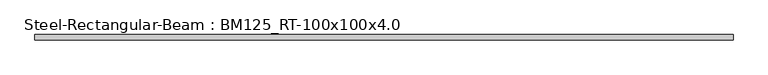
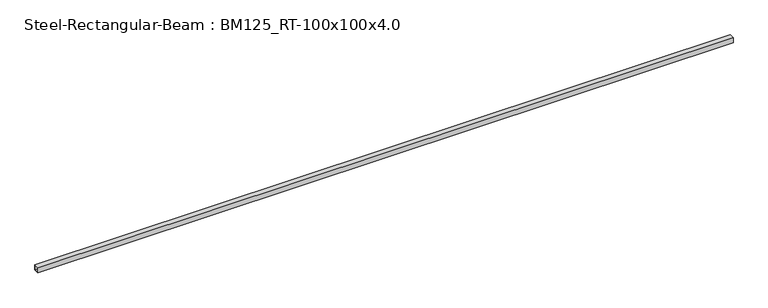
"""IFC4 building model written with IfcOpenShell, lengths in millimetres: beam geometry, Steel-Rectangular-Beam : BM125_RT-100x100x4.0."""

import ifcopenshell
import ifcopenshell.guid

model = None  # the IFC model being written
_history = None  # IfcOwnerHistory: only IFC2X3 demands one
_inside = {}  # id of a spatial element -> (the spatial element, [elements in it])
_under = {}  # id of a project, library or spatial element -> (it, [spatial elements below it])
_declared = {}  # id of a project -> (the project, [libraries it declares])
_typed = {}  # id of a type object -> (the type object, [elements of that type])
_made_of = {}  # id of a material, layer set ... -> (it, [elements and type objects made of it])


def new_model(schema):
    """Start an empty IFC model of exactly this schema.

    Asked for "IFC4X3", IfcOpenShell would pick the latest addendum, in which some entities
    have other attributes; the version numbers below select the first issue.
    IFC2X3 requires an IfcOwnerHistory on every rooted entity: one is made here for all.
    """
    global model, _history
    if schema == "IFC4X3":
        model = ifcopenshell.file(schema_version=(4, 3, 0, 0))
    else:
        model = ifcopenshell.file(schema=schema)
    _inside.clear()
    _under.clear()
    _declared.clear()
    _typed.clear()
    _made_of.clear()
    _history = None
    if model.schema == "IFC2X3":
        org = make("IfcOrganization", Name="unknown")
        user = make(
            "IfcPersonAndOrganization",
            ThePerson=make("IfcPerson", FamilyName="unknown"),
            TheOrganization=org,
        )
        app = make(
            "IfcApplication",
            ApplicationDeveloper=org,
            Version="unknown",
            ApplicationFullName="unknown",
            ApplicationIdentifier="unknown",
        )
        _history = make(
            "IfcOwnerHistory",
            OwningUser=user,
            OwningApplication=app,
            ChangeAction="ADDED",
            CreationDate=0,
        )
    return model


def make(cls, **values):
    """One entity of the class cls with the attributes given. An attribute that is None is left unset."""
    return model.create_entity(
        cls, **{name: value for name, value in values.items() if value is not None}
    )


def rooted(cls, **values):
    """An entity with a GlobalId (a new one), such as an element, a storey or a relation."""
    return make(cls, GlobalId=ifcopenshell.guid.new(), OwnerHistory=_history, **values)


def si_unit(unit_type, name, prefix=None):
    """IfcSIUnit, for example si_unit("LENGTHUNIT", "METRE", prefix="MILLI")."""
    return make("IfcSIUnit", UnitType=unit_type, Prefix=prefix, Name=name)


def assignment(units):
    """IfcUnitAssignment: the units of a project."""
    return None if units is None else make("IfcUnitAssignment", Units=units)


def point(xyz):
    """IfcCartesianPoint."""
    return None if xyz is None else make("IfcCartesianPoint", Coordinates=xyz)


def direction(xyz):
    """IfcDirection."""
    return None if xyz is None else make("IfcDirection", DirectionRatios=xyz)


def frame(location, z_axis=None, x_axis=None):
    """IfcAxis2Placement3D, a coordinate frame: its origin and axes. An axis left out is left unset."""
    return make(
        "IfcAxis2Placement3D",
        Location=point(location),
        Axis=direction(z_axis),
        RefDirection=direction(x_axis),
    )


def origin():
    """The frame at (0, 0, 0) with its axes left unset."""
    return frame((0.0, 0.0, 0.0))


def place(relative_to, where):
    """IfcLocalPlacement: puts the frame where relative to a parent placement (None: the world)."""
    return make(
        "IfcLocalPlacement", PlacementRelTo=relative_to, RelativePlacement=where
    )


def context(
    kind, dimensions, precision=None, world=None, true_north=None, identifier=None
):
    """IfcGeometricRepresentationContext, for example the 3D "Model" context."""
    return make(
        "IfcGeometricRepresentationContext",
        ContextIdentifier=identifier,
        ContextType=kind,
        CoordinateSpaceDimension=dimensions,
        Precision=precision,
        WorldCoordinateSystem=world,
        TrueNorth=true_north,
    )


def project(units=None, contexts=None):
    """IfcProject with its units and contexts."""
    return rooted(
        "IfcProject",
        Name="project",
        RepresentationContexts=contexts,
        UnitsInContext=assignment(units),
    )


def spatial(cls, under=None, at=None, **own):
    """A site, building, storey or space (cls), placed at a placement, below another one or the project."""
    s = rooted(cls, ObjectPlacement=at, **own)
    if under is not None:
        _under.setdefault(under.id(), (under, []))[1].append(s)
    return s


def polyline(points):
    """IfcPolyline through the points."""
    return make("IfcPolyline", Points=[point(p) for p in points])


def outline(outer, holes=None, kind="AREA"):
    """IfcArbitraryClosedProfileDef: a profile drawn as a closed curve; with holes, ...WithVoids."""
    if holes is None:
        return make("IfcArbitraryClosedProfileDef", ProfileType=kind, OuterCurve=outer)
    return make(
        "IfcArbitraryProfileDefWithVoids",
        ProfileType=kind,
        OuterCurve=outer,
        InnerCurves=holes,
    )


def extrude(swept, where, along, depth):
    """IfcExtrudedAreaSolid: the profile swept, set in the frame where, extruded along a direction by depth."""
    return make(
        "IfcExtrudedAreaSolid",
        SweptArea=swept,
        Position=where,
        ExtrudedDirection=direction(along),
        Depth=depth,
    )


def shape(context_of_items, identifier, shape_type, items):
    """IfcShapeRepresentation: the items that make up one representation, for example the "Body"."""
    return make(
        "IfcShapeRepresentation",
        ContextOfItems=context_of_items,
        RepresentationIdentifier=identifier,
        RepresentationType=shape_type,
        Items=items,
    )


def source(mapping_origin, context_of_items, identifier, shape_type, items):
    """IfcRepresentationMap: a shape defined once, which mapped items show again and again."""
    return make(
        "IfcRepresentationMap",
        MappingOrigin=mapping_origin,
        MappedRepresentation=shape(context_of_items, identifier, shape_type, items),
    )


def transform(
    local_origin,
    x_axis=None,
    y_axis=None,
    z_axis=None,
    scale=None,
    scale2=None,
    scale3=None,
    uniform=True,
):
    """IfcCartesianTransformationOperator3D, or its non-uniform kind. x_axis, y_axis, z_axis: its Axis1, 2, 3."""
    if uniform:
        return make(
            "IfcCartesianTransformationOperator3D",
            Axis1=direction(x_axis),
            Axis2=direction(y_axis),
            LocalOrigin=point(local_origin),
            Scale=scale,
            Axis3=direction(z_axis),
        )
    return make(
        "IfcCartesianTransformationOperator3DnonUniform",
        Axis1=direction(x_axis),
        Axis2=direction(y_axis),
        LocalOrigin=point(local_origin),
        Scale=scale,
        Axis3=direction(z_axis),
        Scale2=scale2,
        Scale3=scale3,
    )


def mapped(mapping_source, mapping_target):
    """IfcMappedItem: shows the shape of a source again, moved by a transform."""
    return make(
        "IfcMappedItem", MappingSource=mapping_source, MappingTarget=mapping_target
    )


def made_of(thing, what):
    """Note that an element or type object is made of a material, layer set ...; save() writes the relation."""
    if what is not None:
        _made_of.setdefault(what.id(), (what, []))[1].append(thing)
    return thing


def element(
    cls,
    number,
    at=None,
    inside=None,
    cuts=None,
    type_object=None,
    material=None,
    context=None,
    identifier="Body",
    shape_type=None,
    held_by="IfcProductDefinitionShape",
    body=None,
    shapes=None,
    **own,
):
    """One element of the class cls, such as IfcWall. Its Tag is "e" and its number.

    at: its placement. inside: the storey or other place that contains it. cuts: it is an
    opening in that element (IfcRelVoidsElement). A single representation is given by context,
    identifier, shape_type and body (its items); several are given by shapes. held_by: the class
    of the entity that holds the representations. save() writes the other relations.
    """
    e = rooted(cls, Tag="e%d" % number, ObjectPlacement=at, **own)
    if body is not None:
        shapes = [shape(context, identifier, shape_type, body)]
    if shapes is not None:
        e.Representation = make(held_by, Representations=shapes)
    if inside is not None:
        _inside.setdefault(inside.id(), (inside, []))[1].append(e)
    if cuts is not None:
        rooted(
            "IfcRelVoidsElement", RelatingBuildingElement=cuts, RelatedOpeningElement=e
        )
    if type_object is not None:
        _typed.setdefault(type_object.id(), (type_object, []))[1].append(e)
    return made_of(e, material)


def aggregate(whole, parts):
    """IfcRelAggregates: a whole, such as a stair, and the parts it consists of."""
    return rooted("IfcRelAggregates", RelatingObject=whole, RelatedObjects=parts)


def save(model, path):
    """Write the relations noted so far, then the file.

    IfcRelAggregates (storeys below a building ...), IfcRelContainedInSpatialStructure (elements
    in a storey), IfcRelDefinesByType, IfcRelAssociatesMaterial and IfcRelDeclares: one each for
    every whole, place, type object, material and project.
    """
    for whole, parts in _under.values():
        aggregate(whole, parts)
    for where, things in _inside.values():
        rooted(
            "IfcRelContainedInSpatialStructure",
            RelatedElements=things,
            RelatingStructure=where,
        )
    for kind, things in _typed.values():
        rooted("IfcRelDefinesByType", RelatedObjects=things, RelatingType=kind)
    for what, things in _made_of.values():
        rooted("IfcRelAssociatesMaterial", RelatedObjects=things, RelatingMaterial=what)
    for by, libraries in _declared.values():
        rooted("IfcRelDeclares", RelatingContext=by, RelatedDefinitions=libraries)
    model.write(path)


def steel_rectangular_beam_bm125_rt_100x100x4_0_2c93a6f0(model_context):
    return source(origin(), model_context, "Body", "SweptSolid", [
        extrude(outline(polyline([(-50.0, 50.0), (50.0, 50.0), (50.0, -50.0), (-50.0, -50.0), (-50.0, 50.0)]), holes=[polyline([(46.0, -46.0), (46.0, 46.0), (-46.0, 46.0), (-46.0, -46.0), (46.0, -46.0)])]), frame((-6550.0, 0.0, 0.0), z_axis=(1.0, 0.0, 0.0), x_axis=(0.0, 1.0, 0.0)), (0.0, 0.0, 1.0), 13100.0),
        extrude(outline(polyline([(-50.0, 50.0), (50.0, 50.0), (50.0, -50.0), (-50.0, -50.0), (-50.0, 50.0)]), holes=[polyline([(46.0, -46.0), (46.0, 46.0), (-46.0, 46.0), (-46.0, -46.0), (46.0, -46.0)])]), frame((-6550.0, 0.0, 0.0), z_axis=(1.0, 0.0, 0.0), x_axis=(0.0, 1.0, 0.0)), (0.0, 0.0, 1.0), 13100.0),
        extrude(outline(polyline([(-50.0, 50.0), (50.0, 50.0), (50.0, -50.0), (-50.0, -50.0), (-50.0, 50.0)]), holes=[polyline([(46.0, -46.0), (46.0, 46.0), (-46.0, 46.0), (-46.0, -46.0), (46.0, -46.0)])]), frame((-6550.0, 0.0, 0.0), z_axis=(1.0, 0.0, 0.0), x_axis=(0.0, 1.0, 0.0)), (0.0, 0.0, 1.0), 13100.0),
        extrude(outline(polyline([(-50.0, 50.0), (50.0, 50.0), (50.0, -50.0), (-50.0, -50.0), (-50.0, 50.0)]), holes=[polyline([(46.0, -46.0), (46.0, 46.0), (-46.0, 46.0), (-46.0, -46.0), (46.0, -46.0)])]), frame((-6550.0, 0.0, 0.0), z_axis=(1.0, 0.0, 0.0), x_axis=(0.0, 1.0, 0.0)), (0.0, 0.0, 1.0), 13100.0),
    ])


if __name__ == "__main__":
    model = new_model("IFC4")
    model_context = context("Model", 3, world=origin())
    ifc_project = project(units=[si_unit("LENGTHUNIT", "METRE", prefix="MILLI")], contexts=[model_context])
    site = spatial("IfcSite", under=ifc_project)
    building = spatial("IfcBuilding", under=site)
    placement = place(None, origin())
    steel_rectangular_beam_bm125_rt_100x100x4_0_shape = steel_rectangular_beam_bm125_rt_100x100x4_0_2c93a6f0(model_context)
    element("IfcBeam", 1, ObjectType="Steel-Rectangular-Beam : BM125_RT-100x100x4.0", at=placement, inside=building, context=model_context, shape_type="MappedRepresentation", body=[
        mapped(steel_rectangular_beam_bm125_rt_100x100x4_0_shape, transform((0.0, 0.0, 0.0), x_axis=(1.0, 0.0, 0.0), y_axis=(0.0, 1.0, 0.0), z_axis=(0.0, 0.0, 1.0))),
    ])
    save(model, "model.ifc")

# Revit data of these elements
# Type "Steel-Rectangular-Beam : BM125_RT-100x100x4.0"
#   t = 4 mm
#   Mass per Unit Length = 11.70 kg/m
#   Surface Area = 0.386 m²/m
#   Sectional Area = 14.95 cm²
#   Length [instance default] = 3000 mm
#   H = 100 mm
#   B = 100 mm
#   hec_material4 [instance default] = none
#   hec_material3 [instance default] = none
#   hec_material2 [instance default] = none
#   hec_material1 [instance default] = none
#   Structural Material [instance default] = none
# Element 1 (IfcBeam, "Steel-Rectangular-Beam : BM125_RT-100x100x4.0")
#   hec_material2 = S01AA010-00001_Main Steel Structure Fabrication Work_Shelter/Building_Steel Painting/Coating_for Non-Fireproofed Steel Surface, Surface Preparation, Primer, Second & Final Coat
#   hec_material1 = S03AA007-00001_Main Steel Structure Erection Work_Girth & Purlin
#   Structural Material = S01AA007-00001_Main Steel Structure Fabrication Work_Shelter/Building_Girth & Purlin
#   Materials on its faces: "S01AA010-00001_Main Steel Structure Fabrication Work_Shelter/Building_Steel Painting/Coating_for Non-Fireproofed Steel Surface, Surface Preparation, Primer, Second & Final Coat"
# Materials
#   "S01AA010-00001_Main Steel Structure Fabrication Work_Shelter/Building_Steel Painting/Coating_for Non-Fireproofed Steel Surface, Surface Preparation, Primer, Second & Final Coat": class "Metal", colour RGB 120 120 120, transparency 0, Description = "Paint finished steel", W00) Work Master Code = "S01AA010-00001", W01) Work Master_Lv1 = "Main Steel Structure Fabrication Work", W02) Work Master_Lv2 = "Shelter/Building", W03) Work Master_Spec.1 = "Steel Painting/Coating", W04) Work Master_Spec.2 = "for Non-Fireproofed Steel Surface, Surface Preparation, Primer, Second & Final Coat", Cost = 0
#   "S03AA007-00001_Main Steel Structure Erection Work_Girth & Purlin": class "Metal", colour RGB 120 120 120, transparency 0, Comments = "(30KG/M>Weight)", Description = "Structural steel 50ksi", W00) Work Master Code = "S03AA007-00001", W01) Work Master_Lv1 = "Main Steel Structure Erection Work", W02) Work Master_Lv2 = "Shelter/Building", W03) Work Master_Spec.1 = "Girth & Purlin", Cost = 0
#   "S01AA007-00001_Main Steel Structure Fabrication Work_Shelter/Building_Girth & Purlin": class "Metal", colour RGB 120 120 120, transparency 0, Comments = "(30KG/M>Weight)", Description = "Structural steel 50ksi", W00) Work Master Code = "S01AA007-00001", W01) Work Master_Lv1 = "Main Steel Structure Fabrication Work", W02) Work Master_Lv2 = "Shelter/Building", W03) Work Master_Spec.1 = "Girth & Purlin", Cost = 0
